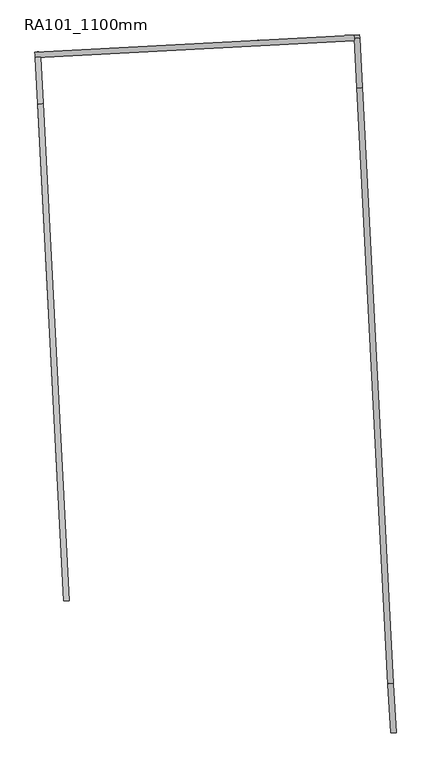
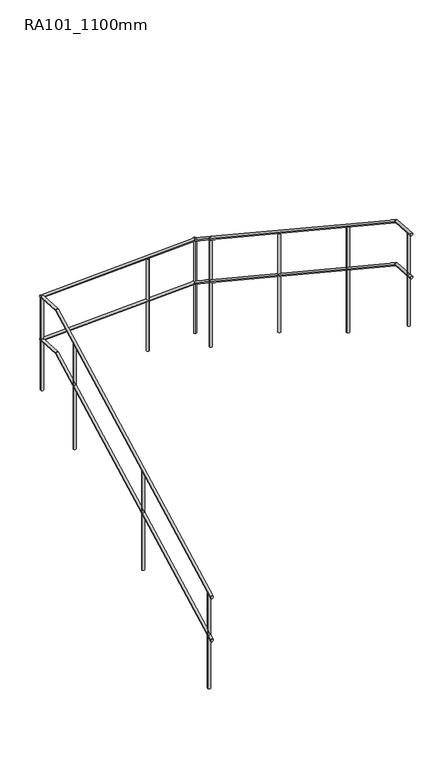
"""IFC4 building model written with IfcOpenShell, lengths in millimetres: railing geometry, RA101_1100mm."""

import ifcopenshell
import ifcopenshell.guid

model = None  # the IFC model being written
_history = None  # IfcOwnerHistory: only IFC2X3 demands one
_inside = {}  # id of a spatial element -> (the spatial element, [elements in it])
_under = {}  # id of a project, library or spatial element -> (it, [spatial elements below it])
_declared = {}  # id of a project -> (the project, [libraries it declares])
_typed = {}  # id of a type object -> (the type object, [elements of that type])
_made_of = {}  # id of a material, layer set ... -> (it, [elements and type objects made of it])


def new_model(schema):
    """Start an empty IFC model of exactly this schema.

    Asked for "IFC4X3", IfcOpenShell would pick the latest addendum, in which some entities
    have other attributes; the version numbers below select the first issue.
    IFC2X3 requires an IfcOwnerHistory on every rooted entity: one is made here for all.
    """
    global model, _history
    if schema == "IFC4X3":
        model = ifcopenshell.file(schema_version=(4, 3, 0, 0))
    else:
        model = ifcopenshell.file(schema=schema)
    _inside.clear()
    _under.clear()
    _declared.clear()
    _typed.clear()
    _made_of.clear()
    _history = None
    if model.schema == "IFC2X3":
        org = make("IfcOrganization", Name="unknown")
        user = make(
            "IfcPersonAndOrganization",
            ThePerson=make("IfcPerson", FamilyName="unknown"),
            TheOrganization=org,
        )
        app = make(
            "IfcApplication",
            ApplicationDeveloper=org,
            Version="unknown",
            ApplicationFullName="unknown",
            ApplicationIdentifier="unknown",
        )
        _history = make(
            "IfcOwnerHistory",
            OwningUser=user,
            OwningApplication=app,
            ChangeAction="ADDED",
            CreationDate=0,
        )
    return model


def make(cls, **values):
    """One entity of the class cls with the attributes given. An attribute that is None is left unset."""
    return model.create_entity(
        cls, **{name: value for name, value in values.items() if value is not None}
    )


def rooted(cls, **values):
    """An entity with a GlobalId (a new one), such as an element, a storey or a relation."""
    return make(cls, GlobalId=ifcopenshell.guid.new(), OwnerHistory=_history, **values)


def si_unit(unit_type, name, prefix=None):
    """IfcSIUnit, for example si_unit("LENGTHUNIT", "METRE", prefix="MILLI")."""
    return make("IfcSIUnit", UnitType=unit_type, Prefix=prefix, Name=name)


def assignment(units):
    """IfcUnitAssignment: the units of a project."""
    return None if units is None else make("IfcUnitAssignment", Units=units)


def point(xyz):
    """IfcCartesianPoint."""
    return None if xyz is None else make("IfcCartesianPoint", Coordinates=xyz)


def direction(xyz):
    """IfcDirection."""
    return None if xyz is None else make("IfcDirection", DirectionRatios=xyz)


def frame(location, z_axis=None, x_axis=None):
    """IfcAxis2Placement3D, a coordinate frame: its origin and axes. An axis left out is left unset."""
    return make(
        "IfcAxis2Placement3D",
        Location=point(location),
        Axis=direction(z_axis),
        RefDirection=direction(x_axis),
    )


def frame_2d(location, x_axis=None):
    """IfcAxis2Placement2D, a coordinate frame in the plane: its origin and x axis."""
    return make(
        "IfcAxis2Placement2D", Location=point(location), RefDirection=direction(x_axis)
    )


def origin():
    """The frame at (0, 0, 0) with its axes left unset."""
    return frame((0.0, 0.0, 0.0))


def place(relative_to, where):
    """IfcLocalPlacement: puts the frame where relative to a parent placement (None: the world)."""
    return make(
        "IfcLocalPlacement", PlacementRelTo=relative_to, RelativePlacement=where
    )


def context(
    kind, dimensions, precision=None, world=None, true_north=None, identifier=None
):
    """IfcGeometricRepresentationContext, for example the 3D "Model" context."""
    return make(
        "IfcGeometricRepresentationContext",
        ContextIdentifier=identifier,
        ContextType=kind,
        CoordinateSpaceDimension=dimensions,
        Precision=precision,
        WorldCoordinateSystem=world,
        TrueNorth=true_north,
    )


def project(units=None, contexts=None):
    """IfcProject with its units and contexts."""
    return rooted(
        "IfcProject",
        Name="project",
        RepresentationContexts=contexts,
        UnitsInContext=assignment(units),
    )


def spatial(cls, under=None, at=None, **own):
    """A site, building, storey or space (cls), placed at a placement, below another one or the project."""
    s = rooted(cls, ObjectPlacement=at, **own)
    if under is not None:
        _under.setdefault(under.id(), (under, []))[1].append(s)
    return s


def circle_curve(where, radius):
    """IfcCircle in the frame where."""
    return make("IfcCircle", Position=where, Radius=radius)


def ellipse_curve(where, semi_axis1, semi_axis2):
    """IfcEllipse in the frame where."""
    return make(
        "IfcEllipse", Position=where, SemiAxis1=semi_axis1, SemiAxis2=semi_axis2
    )


def trimmed(basis, trim1, trim2, sense, master):
    """IfcTrimmedCurve: the piece of a basis curve between two trims."""
    return make(
        "IfcTrimmedCurve",
        BasisCurve=basis,
        Trim1=trim1,
        Trim2=trim2,
        SenseAgreement=sense,
        MasterRepresentation=master,
    )


def segment(curve, same_sense, transition):
    """IfcCompositeCurveSegment."""
    return make(
        "IfcCompositeCurveSegment",
        Transition=transition,
        SameSense=same_sense,
        ParentCurve=curve,
    )


def composite_curve(segments, self_intersect=None):
    """IfcCompositeCurve: segments joined end to end."""
    return make("IfcCompositeCurve", Segments=segments, SelfIntersect=self_intersect)


def outline(outer, holes=None, kind="AREA"):
    """IfcArbitraryClosedProfileDef: a profile drawn as a closed curve; with holes, ...WithVoids."""
    if holes is None:
        return make("IfcArbitraryClosedProfileDef", ProfileType=kind, OuterCurve=outer)
    return make(
        "IfcArbitraryProfileDefWithVoids",
        ProfileType=kind,
        OuterCurve=outer,
        InnerCurves=holes,
    )


def extrude(swept, where, along, depth):
    """IfcExtrudedAreaSolid: the profile swept, set in the frame where, extruded along a direction by depth."""
    return make(
        "IfcExtrudedAreaSolid",
        SweptArea=swept,
        Position=where,
        ExtrudedDirection=direction(along),
        Depth=depth,
    )


def shape(context_of_items, identifier, shape_type, items):
    """IfcShapeRepresentation: the items that make up one representation, for example the "Body"."""
    return make(
        "IfcShapeRepresentation",
        ContextOfItems=context_of_items,
        RepresentationIdentifier=identifier,
        RepresentationType=shape_type,
        Items=items,
    )


def source(mapping_origin, context_of_items, identifier, shape_type, items):
    """IfcRepresentationMap: a shape defined once, which mapped items show again and again."""
    return make(
        "IfcRepresentationMap",
        MappingOrigin=mapping_origin,
        MappedRepresentation=shape(context_of_items, identifier, shape_type, items),
    )


def transform(
    local_origin,
    x_axis=None,
    y_axis=None,
    z_axis=None,
    scale=None,
    scale2=None,
    scale3=None,
    uniform=True,
):
    """IfcCartesianTransformationOperator3D, or its non-uniform kind. x_axis, y_axis, z_axis: its Axis1, 2, 3."""
    if uniform:
        return make(
            "IfcCartesianTransformationOperator3D",
            Axis1=direction(x_axis),
            Axis2=direction(y_axis),
            LocalOrigin=point(local_origin),
            Scale=scale,
            Axis3=direction(z_axis),
        )
    return make(
        "IfcCartesianTransformationOperator3DnonUniform",
        Axis1=direction(x_axis),
        Axis2=direction(y_axis),
        LocalOrigin=point(local_origin),
        Scale=scale,
        Axis3=direction(z_axis),
        Scale2=scale2,
        Scale3=scale3,
    )


def mapped(mapping_source, mapping_target):
    """IfcMappedItem: shows the shape of a source again, moved by a transform."""
    return make(
        "IfcMappedItem", MappingSource=mapping_source, MappingTarget=mapping_target
    )


def made_of(thing, what):
    """Note that an element or type object is made of a material, layer set ...; save() writes the relation."""
    if what is not None:
        _made_of.setdefault(what.id(), (what, []))[1].append(thing)
    return thing


def element(
    cls,
    number,
    at=None,
    inside=None,
    cuts=None,
    type_object=None,
    material=None,
    context=None,
    identifier="Body",
    shape_type=None,
    held_by="IfcProductDefinitionShape",
    body=None,
    shapes=None,
    **own,
):
    """One element of the class cls, such as IfcWall. Its Tag is "e" and its number.

    at: its placement. inside: the storey or other place that contains it. cuts: it is an
    opening in that element (IfcRelVoidsElement). A single representation is given by context,
    identifier, shape_type and body (its items); several are given by shapes. held_by: the class
    of the entity that holds the representations. save() writes the other relations.
    """
    e = rooted(cls, Tag="e%d" % number, ObjectPlacement=at, **own)
    if body is not None:
        shapes = [shape(context, identifier, shape_type, body)]
    if shapes is not None:
        e.Representation = make(held_by, Representations=shapes)
    if inside is not None:
        _inside.setdefault(inside.id(), (inside, []))[1].append(e)
    if cuts is not None:
        rooted(
            "IfcRelVoidsElement", RelatingBuildingElement=cuts, RelatedOpeningElement=e
        )
    if type_object is not None:
        _typed.setdefault(type_object.id(), (type_object, []))[1].append(e)
    return made_of(e, material)


def aggregate(whole, parts):
    """IfcRelAggregates: a whole, such as a stair, and the parts it consists of."""
    return rooted("IfcRelAggregates", RelatingObject=whole, RelatedObjects=parts)


def save(model, path):
    """Write the relations noted so far, then the file.

    IfcRelAggregates (storeys below a building ...), IfcRelContainedInSpatialStructure (elements
    in a storey), IfcRelDefinesByType, IfcRelAssociatesMaterial and IfcRelDeclares: one each for
    every whole, place, type object, material and project.
    """
    for whole, parts in _under.values():
        aggregate(whole, parts)
    for where, things in _inside.values():
        rooted(
            "IfcRelContainedInSpatialStructure",
            RelatedElements=things,
            RelatingStructure=where,
        )
    for kind, things in _typed.values():
        rooted("IfcRelDefinesByType", RelatedObjects=things, RelatingType=kind)
    for what, things in _made_of.values():
        rooted("IfcRelAssociatesMaterial", RelatedObjects=things, RelatingMaterial=what)
    for by, libraries in _declared.values():
        rooted("IfcRelDeclares", RelatingContext=by, RelatedDefinitions=libraries)
    model.write(path)


def plane_surface(at):
    """IfcPlane: the flat surface through the origin of the frame at, square to its z axis."""
    return make("IfcPlane", Position=at)


def cylinder_surface(at, radius):
    """IfcCylindricalSurface: all points at the distance radius from the z axis of the frame at."""
    return make("IfcCylindricalSurface", Position=at, Radius=radius)


def advanced_brep(points, edges, surfaces, faces):
    """IfcAdvancedBrep: a solid bounded by faces that lie on surfaces and meet in shared edges.

    An edge is (start, end): straight between two places in points (the first is 0);
    or (start, end, curve); or (start, end, curve, False) where it runs against its curve.
    A face is (place in surfaces, loops), or (place, loops, False) where it looks against
    its surface's normal. A loop lists edges by number (the first is 1), with a minus sign
    where the edge is run from its end to its start. The first loop is the outer one.
    """
    corners = [point(p) for p in points]
    vertices = [make("IfcVertexPoint", VertexGeometry=c) for c in corners]
    made = []
    for start, end, *more in edges:
        made.append(
            make(
                "IfcEdgeCurve",
                EdgeStart=vertices[start],
                EdgeEnd=vertices[end],
                EdgeGeometry=more[0] if more else make("IfcPolyline", Points=[corners[start], corners[end]]),
                SameSense=more[1] if len(more) > 1 else True,
            )
        )
    hull = []
    for where, loops, *sense in faces:
        bounds = []
        for j, loop in enumerate(loops):
            ring = [make("IfcOrientedEdge", EdgeElement=made[abs(k) - 1], Orientation=k > 0) for k in loop]
            bounds.append(
                make(
                    "IfcFaceOuterBound" if j == 0 else "IfcFaceBound",
                    Bound=make("IfcEdgeLoop", EdgeList=ring),
                    Orientation=True,
                )
            )
        hull.append(make("IfcAdvancedFace", Bounds=bounds, FaceSurface=surfaces[where], SameSense=sense[0] if sense else True))
    return make("IfcAdvancedBrep", Outer=make("IfcClosedShell", CfsFaces=hull))


def ra101_1100mm_54c19647(model_context):
    return source(origin(), model_context, "Body", "SolidModel", [
        advanced_brep(
        [(22896.1789103, 12534.7141331, 457.1248327), (22926.1377964, 12536.2842117, 457.1248327), (22754.6396676, 15235.4437699, 2210.0), (22784.5985536, 15237.0138486, 2210.0), (22741.5052252, 15486.0638601, 2210.0), (22771.4641113, 15487.6339388, 2210.0)],
        [
            (0, 1, ellipse_curve(frame((22911.1583533, 12535.4991724, 457.1248327), z_axis=(0.05233595624294174, -0.998629534754574, 0.0), x_axis=(0.0, 0.0, -0.9999999999999999)), 17.8751673, 15.0)),
            (1, 0, ellipse_curve(frame((22911.1583533, 12535.4991724, 457.1248327), z_axis=(0.05233595624294174, -0.998629534754574, 0.0), x_axis=(0.0, 0.0, -0.9999999999999999)), 17.8751673, 15.0)),
            (0, 2),
            (2, 3, ellipse_curve(frame((22769.6191106, 15236.2288092, 2210.0), z_axis=(0.05018733030882238, -0.9576313096148807, -0.28359038545367066), x_axis=(-0.014841974004015643, 0.28320173468646914, -0.9589455111101144)), 15.6421818, 15.0)),
            (3, 1),
            (3, 2, ellipse_curve(frame((22769.6191106, 15236.2288092, 2210.0), z_axis=(0.05018733030882238, -0.9576313096148807, -0.28359038545367066), x_axis=(-0.014841974004015643, 0.28320173468646914, -0.9589455111101144)), 15.6421818, 15.0)),
            (4, 5, circle_curve(frame((22756.4846683, 15486.8488994, 2210.0), z_axis=(-0.05233595624293797, 0.9986295347545743, 0.0), x_axis=(0.9986295347545743, 0.05233595624293797, 0.0)), 15.0)),
            (5, 4, circle_curve(frame((22756.4846683, 15486.8488994, 2210.0), z_axis=(-0.05233595624293797, 0.9986295347545743, 0.0), x_axis=(0.9986295347545743, 0.05233595624293797, 0.0)), 15.0)),
            (2, 4),
            (5, 3),
        ],
        [
            plane_surface(frame((22911.1583533, 12535.4991724, 475.0), z_axis=(0.05233595624294174, -0.998629534754574, 0.0), x_axis=(0.998629534754574, 0.05233595624294174, 0.0))),
            cylinder_surface(frame((22910.731374, 12543.6464234, 462.4127052), z_axis=(0.04391787398555367, -0.8380029565528062, -0.5438954542495689), x_axis=(0.998629534754574, 0.052335956242941746, 0.0)), 15.0),
            plane_surface(frame((22756.4846683, 15486.8488994, 2225.0), z_axis=(-0.05233595624294184, 0.998629534754574, 0.0), x_axis=(0.998629534754574, 0.05233595624294184, 0.0))),
            cylinder_surface(frame((22769.8512715, 15231.7989162, 2210.0), z_axis=(0.05233595624293797, -0.9986295347545743, 0.0), x_axis=(0.9986295347545743, 0.05233595624293797, 0.0)), 15.0),
        ],
        [
            (0, [[1, 2]]),
            (1, [[-1, 3, 4, 5]]),
            (1, [[-2, -5, 6, -3]]),
            (2, [[7, 8]]),
            (3, [[-4, 9, -8, 10]]),
            (3, [[-6, -10, -7, -9]]),
        ],
    ),
        advanced_brep(
        [(22739.9351465, 15516.0227461, 2210.0), (22741.5052252, 15486.0638601, 2210.0), (24475.8528668, 15606.9983388, 2210.0), (24477.4229455, 15577.0394528, 2210.0)],
        [
            (0, 1, circle_curve(frame((22740.7201859, 15501.0433031, 2210.0), z_axis=(-0.998629534754574, -0.05233595624294185, 0.0), x_axis=(0.05233595624294185, -0.998629534754574, 0.0)), 15.0)),
            (1, 0, circle_curve(frame((22740.7201859, 15501.0433031, 2210.0), z_axis=(-0.998629534754574, -0.05233595624294185, 0.0), x_axis=(0.05233595624294185, -0.998629534754574, 0.0)), 15.0)),
            (2, 3, circle_curve(frame((24476.6379061, 15592.0188958, 2210.0), z_axis=(0.998629534754574, 0.05233595624294185, 0.0), x_axis=(0.05233595624294185, -0.998629534754574, 0.0)), 15.0)),
            (3, 2, circle_curve(frame((24476.6379061, 15592.0188958, 2210.0), z_axis=(0.998629534754574, 0.05233595624294185, 0.0), x_axis=(0.05233595624294185, -0.998629534754574, 0.0)), 15.0)),
            (0, 2),
            (3, 1),
        ],
        [
            plane_surface(frame((22740.7201859, 15501.0433031, 2225.0), z_axis=(-0.9986295347545743, -0.052335956242937944, 0.0), x_axis=(0.052335956242937944, -0.9986295347545743, 0.0))),
            plane_surface(frame((24476.6379061, 15592.0188958, 2225.0), z_axis=(0.9986295347545743, 0.052335956242937104, 0.0), x_axis=(0.052335956242937104, -0.9986295347545743, 0.0))),
            cylinder_surface(frame((22740.7201859, 15501.0433031, 2210.0), z_axis=(-0.998629534754574, -0.05233595624294185, 0.0), x_axis=(0.05233595624294185, -0.998629534754574, 0.0)), 15.0),
        ],
        [
            (0, [[1, 2]]),
            (1, [[3, 4]]),
            (2, [[-1, 5, -4, 6]]),
            (2, [[-2, -6, -3, -5]]),
        ],
    ),
        advanced_brep(
        [(24505.8117528, 15608.5684175, 2210.0), (24475.8528668, 15606.9983388, 2210.0), (24506.8498874, 15588.7596297, 2210.0), (24476.8910014, 15587.189551, 2210.0), (24520.7484348, 15323.5595483, 2382.1248327), (24490.7895487, 15321.9894696, 2382.1248327)],
        [
            (0, 1, circle_curve(frame((24490.8323098, 15607.7833782, 2210.0), z_axis=(-0.052335956242937104, 0.9986295347545743, 0.0), x_axis=(-0.9986295347545743, -0.052335956242937104, 0.0)), 15.0)),
            (1, 0, circle_curve(frame((24490.8323098, 15607.7833782, 2210.0), z_axis=(-0.052335956242937104, 0.9986295347545743, 0.0), x_axis=(-0.9986295347545743, -0.052335956242937104, 0.0)), 15.0)),
            (0, 2),
            (2, 3, ellipse_curve(frame((24491.8704444, 15587.9745903, 2210.0), z_axis=(-0.050187330308819895, 0.9576313096148807, -0.28359038545367116), x_axis=(-0.014841974004020982, 0.2832017346864703, 0.9589455111101142)), 15.6421818, 15.0)),
            (3, 1),
            (3, 2, ellipse_curve(frame((24491.8704444, 15587.9745903, 2210.0), z_axis=(-0.050187330308819895, 0.9576313096148807, -0.28359038545367116), x_axis=(-0.014841974004020982, 0.2832017346864703, 0.9589455111101142)), 15.6421818, 15.0)),
            (4, 5, ellipse_curve(frame((24505.7689917, 15322.774509, 2382.1248327), z_axis=(0.052335956242937104, -0.9986295347545743, 0.0), x_axis=(0.0, 0.0, -1.0)), 17.8751673, 15.0)),
            (5, 4, ellipse_curve(frame((24505.7689917, 15322.774509, 2382.1248327), z_axis=(0.052335956242937104, -0.9986295347545743, 0.0), x_axis=(0.0, 0.0, -1.0)), 17.8751673, 15.0)),
            (2, 4),
            (5, 3),
        ],
        [
            plane_surface(frame((24490.8323098, 15607.7833782, 2225.0), z_axis=(-0.05233595624294184, 0.998629534754574, 0.0), x_axis=(0.998629534754574, 0.05233595624294184, 0.0))),
            cylinder_surface(frame((24490.8323098, 15607.7833782, 2210.0), z_axis=(-0.052335956242937104, 0.9986295347545743, 0.0), x_axis=(-0.9986295347545743, -0.052335956242937104, 0.0)), 15.0),
            plane_surface(frame((24505.7689917, 15322.774509, 2400.0), z_axis=(0.052335956242937104, -0.9986295347545743, 0.0), x_axis=(0.9986295347545743, 0.052335956242937104, 0.0))),
            cylinder_surface(frame((24492.0652629, 15584.2572324, 2212.4127052), z_axis=(-0.04391787398554974, 0.8380029565528057, -0.5438954542495701), x_axis=(-0.9986295347545743, -0.0523359562429371, 0.0)), 15.0),
        ],
        [
            (0, [[1, 2]]),
            (1, [[-1, 3, 4, 5]]),
            (1, [[-2, -5, 6, -3]]),
            (2, [[7, 8]]),
            (3, [[-4, 9, -8, 10]]),
            (3, [[-6, -10, -7, -9]]),
        ],
    ),
        advanced_brep(
        [(24520.7484348, 15323.5595483, 2382.1248327), (24490.7895487, 15321.9894696, 2382.1248327), (24690.5490938, 12083.5699627, 4485.0), (24660.5902078, 12081.999884, 4485.0), (24704.4476412, 11818.3698813, 4485.0), (24674.4887551, 11816.7998026, 4485.0)],
        [
            (0, 1, ellipse_curve(frame((24505.7689917, 15322.774509, 2382.1248327), z_axis=(-0.05233595624294191, 0.998629534754574, 0.0), x_axis=(0.0, 0.0, -1.0)), 17.8751673, 15.0)),
            (1, 0, ellipse_curve(frame((24505.7689917, 15322.774509, 2382.1248327), z_axis=(-0.05233595624294191, 0.998629534754574, 0.0), x_axis=(0.0, 0.0, -1.0)), 17.8751673, 15.0)),
            (0, 2),
            (2, 3, ellipse_curve(frame((24675.5696508, 12082.7849234, 4485.0), z_axis=(-0.05018733030882025, 0.9576313096148807, -0.28359038545367127), x_axis=(0.014841974004007963, -0.28320173468647103, -0.9589455111101143)), 15.6421818, 15.0)),
            (3, 1),
            (3, 2, ellipse_curve(frame((24675.5696508, 12082.7849234, 4485.0), z_axis=(-0.05018733030882025, 0.9576313096148807, -0.28359038545367127), x_axis=(0.014841974004007963, -0.28320173468647103, -0.9589455111101143)), 15.6421818, 15.0)),
            (4, 5, circle_curve(frame((24689.4681982, 11817.584842, 4485.0), z_axis=(0.05233595624293375, -0.9986295347545745, 0.0), x_axis=(-0.9986295347545745, -0.05233595624293375, 0.0)), 15.0)),
            (5, 4, circle_curve(frame((24689.4681982, 11817.584842, 4485.0), z_axis=(0.05233595624293375, -0.9986295347545745, 0.0), x_axis=(-0.9986295347545745, -0.05233595624293375, 0.0)), 15.0)),
            (2, 4),
            (5, 3),
        ],
        [
            plane_surface(frame((24505.7689917, 15322.774509, 2400.0), z_axis=(-0.05233595624294191, 0.998629534754574, 0.0), x_axis=(0.998629534754574, 0.05233595624294191, 0.0))),
            cylinder_surface(frame((24506.1959711, 15314.627258, 2387.4127052), z_axis=(-0.04391787398555378, 0.8380029565528053, -0.5438954542495702), x_axis=(-0.998629534754574, -0.052335956242941926, 0.0)), 15.0),
            plane_surface(frame((24689.4681982, 11817.584842, 4500.0), z_axis=(0.05233595624293375, -0.9986295347545745, 0.0), x_axis=(0.9986295347545745, 0.05233595624293375, 0.0))),
            cylinder_surface(frame((24675.33749, 12087.2148164, 4485.0), z_axis=(-0.05233595624293375, 0.9986295347545745, 0.0), x_axis=(-0.9986295347545745, -0.05233595624293375, 0.0)), 15.0),
        ],
        [
            (0, [[1, 2]]),
            (1, [[-1, 3, 4, 5]]),
            (1, [[-2, -5, 6, -3]]),
            (2, [[7, 8]]),
            (3, [[-4, 9, -8, 10]]),
            (3, [[-6, -10, -7, -9]]),
        ],
    ),
        advanced_brep(
        [(22896.1789103, 12534.7141331, 957.1248327), (22926.1377964, 12536.2842117, 957.1248327), (22754.6396676, 15235.4437699, 2710.0), (22784.5985536, 15237.0138486, 2710.0), (22741.5052252, 15486.0638601, 2710.0), (22771.4641113, 15487.6339388, 2710.0)],
        [
            (0, 1, ellipse_curve(frame((22911.1583533, 12535.4991724, 957.1248327), z_axis=(0.05233595624294174, -0.998629534754574, 0.0), x_axis=(0.0, 0.0, -0.9999999999999999)), 17.8751673, 15.0)),
            (1, 0, ellipse_curve(frame((22911.1583533, 12535.4991724, 957.1248327), z_axis=(0.05233595624294174, -0.998629534754574, 0.0), x_axis=(0.0, 0.0, -0.9999999999999999)), 17.8751673, 15.0)),
            (0, 2),
            (2, 3, ellipse_curve(frame((22769.6191106, 15236.2288092, 2710.0), z_axis=(0.05018733030882238, -0.9576313096148807, -0.28359038545367066), x_axis=(-0.014841974004015643, 0.28320173468646914, -0.9589455111101144)), 15.6421818, 15.0)),
            (3, 1),
            (3, 2, ellipse_curve(frame((22769.6191106, 15236.2288092, 2710.0), z_axis=(0.05018733030882238, -0.9576313096148807, -0.28359038545367066), x_axis=(-0.014841974004015643, 0.28320173468646914, -0.9589455111101144)), 15.6421818, 15.0)),
            (4, 5, circle_curve(frame((22756.4846683, 15486.8488994, 2710.0), z_axis=(-0.05233595624293797, 0.9986295347545743, 0.0), x_axis=(0.9986295347545743, 0.05233595624293797, 0.0)), 15.0)),
            (5, 4, circle_curve(frame((22756.4846683, 15486.8488994, 2710.0), z_axis=(-0.05233595624293797, 0.9986295347545743, 0.0), x_axis=(0.9986295347545743, 0.05233595624293797, 0.0)), 15.0)),
            (2, 4),
            (5, 3),
        ],
        [
            plane_surface(frame((22911.1583533, 12535.4991724, 975.0), z_axis=(0.05233595624294174, -0.998629534754574, 0.0), x_axis=(0.998629534754574, 0.05233595624294174, 0.0))),
            cylinder_surface(frame((22910.731374, 12543.6464234, 962.4127052), z_axis=(0.04391787398555367, -0.8380029565528062, -0.5438954542495689), x_axis=(0.998629534754574, 0.052335956242941746, 0.0)), 15.0),
            plane_surface(frame((22756.4846683, 15486.8488994, 2725.0), z_axis=(-0.05233595624294184, 0.998629534754574, 0.0), x_axis=(0.998629534754574, 0.05233595624294184, 0.0))),
            cylinder_surface(frame((22769.8512715, 15231.7989162, 2710.0), z_axis=(0.05233595624293797, -0.9986295347545743, 0.0), x_axis=(0.9986295347545743, 0.05233595624293797, 0.0)), 15.0),
        ],
        [
            (0, [[1, 2]]),
            (1, [[-1, 3, 4, 5]]),
            (1, [[-2, -5, 6, -3]]),
            (2, [[7, 8]]),
            (3, [[-4, 9, -8, 10]]),
            (3, [[-6, -10, -7, -9]]),
        ],
    ),
        advanced_brep(
        [(22739.9351465, 15516.0227461, 2710.0), (22741.5052252, 15486.0638601, 2710.0), (24475.8528668, 15606.9983388, 2710.0), (24477.4229455, 15577.0394528, 2710.0)],
        [
            (0, 1, circle_curve(frame((22740.7201859, 15501.0433031, 2710.0), z_axis=(-0.998629534754574, -0.05233595624294185, 0.0), x_axis=(0.05233595624294185, -0.998629534754574, 0.0)), 15.0)),
            (1, 0, circle_curve(frame((22740.7201859, 15501.0433031, 2710.0), z_axis=(-0.998629534754574, -0.05233595624294185, 0.0), x_axis=(0.05233595624294185, -0.998629534754574, 0.0)), 15.0)),
            (2, 3, circle_curve(frame((24476.6379061, 15592.0188958, 2710.0), z_axis=(0.998629534754574, 0.05233595624294185, 0.0), x_axis=(0.05233595624294185, -0.998629534754574, 0.0)), 15.0)),
            (3, 2, circle_curve(frame((24476.6379061, 15592.0188958, 2710.0), z_axis=(0.998629534754574, 0.05233595624294185, 0.0), x_axis=(0.05233595624294185, -0.998629534754574, 0.0)), 15.0)),
            (0, 2),
            (3, 1),
        ],
        [
            plane_surface(frame((22740.7201859, 15501.0433031, 2725.0), z_axis=(-0.9986295347545743, -0.052335956242937944, 0.0), x_axis=(0.052335956242937944, -0.9986295347545743, 0.0))),
            plane_surface(frame((24476.6379061, 15592.0188958, 2725.0), z_axis=(0.9986295347545743, 0.052335956242937104, 0.0), x_axis=(0.052335956242937104, -0.9986295347545743, 0.0))),
            cylinder_surface(frame((22740.7201859, 15501.0433031, 2710.0), z_axis=(-0.998629534754574, -0.05233595624294185, 0.0), x_axis=(0.05233595624294185, -0.998629534754574, 0.0)), 15.0),
        ],
        [
            (0, [[1, 2]]),
            (1, [[3, 4]]),
            (2, [[-1, 5, -4, 6]]),
            (2, [[-2, -6, -3, -5]]),
        ],
    ),
        advanced_brep(
        [(24505.8117528, 15608.5684175, 2710.0), (24475.8528668, 15606.9983388, 2710.0), (24506.8498874, 15588.7596297, 2710.0), (24476.8910014, 15587.189551, 2710.0), (24520.7484348, 15323.5595483, 2882.1248327), (24490.7895487, 15321.9894696, 2882.1248327)],
        [
            (0, 1, circle_curve(frame((24490.8323098, 15607.7833782, 2710.0), z_axis=(-0.052335956242937104, 0.9986295347545743, 0.0), x_axis=(-0.9986295347545743, -0.052335956242937104, 0.0)), 15.0)),
            (1, 0, circle_curve(frame((24490.8323098, 15607.7833782, 2710.0), z_axis=(-0.052335956242937104, 0.9986295347545743, 0.0), x_axis=(-0.9986295347545743, -0.052335956242937104, 0.0)), 15.0)),
            (0, 2),
            (2, 3, ellipse_curve(frame((24491.8704444, 15587.9745903, 2710.0), z_axis=(-0.050187330308819895, 0.9576313096148807, -0.28359038545367116), x_axis=(-0.014841974004020982, 0.2832017346864703, 0.9589455111101142)), 15.6421818, 15.0)),
            (3, 1),
            (3, 2, ellipse_curve(frame((24491.8704444, 15587.9745903, 2710.0), z_axis=(-0.050187330308819895, 0.9576313096148807, -0.28359038545367116), x_axis=(-0.014841974004020982, 0.2832017346864703, 0.9589455111101142)), 15.6421818, 15.0)),
            (4, 5, ellipse_curve(frame((24505.7689917, 15322.774509, 2882.1248327), z_axis=(0.052335956242937104, -0.9986295347545743, 0.0), x_axis=(0.0, 0.0, -1.0)), 17.8751673, 15.0)),
            (5, 4, ellipse_curve(frame((24505.7689917, 15322.774509, 2882.1248327), z_axis=(0.052335956242937104, -0.9986295347545743, 0.0), x_axis=(0.0, 0.0, -1.0)), 17.8751673, 15.0)),
            (2, 4),
            (5, 3),
        ],
        [
            plane_surface(frame((24490.8323098, 15607.7833782, 2725.0), z_axis=(-0.05233595624294184, 0.998629534754574, 0.0), x_axis=(0.998629534754574, 0.05233595624294184, 0.0))),
            cylinder_surface(frame((24490.8323098, 15607.7833782, 2710.0), z_axis=(-0.052335956242937104, 0.9986295347545743, 0.0), x_axis=(-0.9986295347545743, -0.052335956242937104, 0.0)), 15.0),
            plane_surface(frame((24505.7689917, 15322.774509, 2900.0), z_axis=(0.052335956242937104, -0.9986295347545743, 0.0), x_axis=(0.9986295347545743, 0.052335956242937104, 0.0))),
            cylinder_surface(frame((24492.0652629, 15584.2572324, 2712.4127052), z_axis=(-0.04391787398554974, 0.8380029565528057, -0.5438954542495701), x_axis=(-0.9986295347545743, -0.0523359562429371, 0.0)), 15.0),
        ],
        [
            (0, [[1, 2]]),
            (1, [[-1, 3, 4, 5]]),
            (1, [[-2, -5, 6, -3]]),
            (2, [[7, 8]]),
            (3, [[-4, 9, -8, 10]]),
            (3, [[-6, -10, -7, -9]]),
        ],
    ),
        advanced_brep(
        [(24520.7484348, 15323.5595483, 2882.1248327), (24490.7895487, 15321.9894696, 2882.1248327), (24690.5490938, 12083.5699627, 4985.0), (24660.5902078, 12081.999884, 4985.0), (24704.4476412, 11818.3698813, 4985.0), (24674.4887551, 11816.7998026, 4985.0)],
        [
            (0, 1, ellipse_curve(frame((24505.7689917, 15322.774509, 2882.1248327), z_axis=(-0.05233595624294191, 0.998629534754574, 0.0), x_axis=(0.0, 0.0, -1.0)), 17.8751673, 15.0)),
            (1, 0, ellipse_curve(frame((24505.7689917, 15322.774509, 2882.1248327), z_axis=(-0.05233595624294191, 0.998629534754574, 0.0), x_axis=(0.0, 0.0, -1.0)), 17.8751673, 15.0)),
            (0, 2),
            (2, 3, ellipse_curve(frame((24675.5696508, 12082.7849234, 4985.0), z_axis=(-0.05018733030882025, 0.9576313096148807, -0.28359038545367127), x_axis=(0.014841974004007963, -0.28320173468647103, -0.9589455111101143)), 15.6421818, 15.0)),
            (3, 1),
            (3, 2, ellipse_curve(frame((24675.5696508, 12082.7849234, 4985.0), z_axis=(-0.05018733030882025, 0.9576313096148807, -0.28359038545367127), x_axis=(0.014841974004007963, -0.28320173468647103, -0.9589455111101143)), 15.6421818, 15.0)),
            (4, 5, circle_curve(frame((24689.4681982, 11817.584842, 4985.0), z_axis=(0.05233595624293375, -0.9986295347545745, 0.0), x_axis=(-0.9986295347545745, -0.05233595624293375, 0.0)), 15.0)),
            (5, 4, circle_curve(frame((24689.4681982, 11817.584842, 4985.0), z_axis=(0.05233595624293375, -0.9986295347545745, 0.0), x_axis=(-0.9986295347545745, -0.05233595624293375, 0.0)), 15.0)),
            (2, 4),
            (5, 3),
        ],
        [
            plane_surface(frame((24505.7689917, 15322.774509, 2900.0), z_axis=(-0.05233595624294191, 0.998629534754574, 0.0), x_axis=(0.998629534754574, 0.05233595624294191, 0.0))),
            cylinder_surface(frame((24506.1959711, 15314.627258, 2887.4127052), z_axis=(-0.04391787398555378, 0.8380029565528053, -0.5438954542495702), x_axis=(-0.998629534754574, -0.052335956242941926, 0.0)), 15.0),
            plane_surface(frame((24689.4681982, 11817.584842, 5000.0), z_axis=(0.05233595624293375, -0.9986295347545745, 0.0), x_axis=(0.9986295347545745, 0.05233595624293375, 0.0))),
            cylinder_surface(frame((24675.33749, 12087.2148164, 4985.0), z_axis=(-0.05233595624293375, 0.9986295347545745, 0.0), x_axis=(-0.9986295347545745, -0.05233595624293375, 0.0)), 15.0),
        ],
        [
            (0, [[1, 2]]),
            (1, [[-1, 3, 4, 5]]),
            (1, [[-2, -5, 6, -3]]),
            (2, [[7, 8]]),
            (3, [[-4, 9, -8, 10]]),
            (3, [[-6, -10, -7, -9]]),
        ],
    ),
        extrude(outline(composite_curve([segment(trimmed(circle_curve(frame_2d((24631.3752867, 12926.0636256)), 15.0), [point((24616.3958437, 12925.2785862))], [point((24646.3547297, 12926.8486649))], False, "CARTESIAN"), True, "CONTINUOUS"), segment(trimmed(circle_curve(frame_2d((24631.3752867, 12926.0636256)), 15.0), [point((24646.3547297, 12926.8486649))], [point((24616.3958437, 12925.2785862))], False, "CARTESIAN"), True, "CONTINUOUS")], self_intersect=False)), frame((0.0, 0.0, 3200.0), z_axis=(0.0, 0.0, 1.0), x_axis=(1.0, 0.0, 0.0)), (0.0, 0.0, 1.0), 1225.5555556),
        extrude(outline(composite_curve([segment(trimmed(circle_curve(frame_2d((24568.5721392, 14124.4190673)), 15.0), [point((24553.5926962, 14123.6340279))], [point((24583.5515823, 14125.2041066))], False, "CARTESIAN"), True, "CONTINUOUS"), segment(trimmed(circle_curve(frame_2d((24568.5721392, 14124.4190673)), 15.0), [point((24583.5515823, 14125.2041066))], [point((24553.5926962, 14123.6340279))], False, "CARTESIAN"), True, "CONTINUOUS")], self_intersect=False)), frame((0.0, 0.0, 2500.0), z_axis=(0.0, 0.0, 1.0), x_axis=(1.0, 0.0, 0.0)), (0.0, 0.0, 1.0), 1147.7777778),
        extrude(outline(composite_curve([segment(trimmed(circle_curve(frame_2d((23954.0550706, 15564.6314899)), 15.0), [point((23954.84011, 15549.6520469))], [point((23953.2700313, 15579.6109329))], False, "CARTESIAN"), True, "CONTINUOUS"), segment(trimmed(circle_curve(frame_2d((23954.0550706, 15564.6314899)), 15.0), [point((23953.2700313, 15579.6109329))], [point((23954.84011, 15549.6520469))], False, "CARTESIAN"), True, "CONTINUOUS")], self_intersect=False)), frame((0.0, 0.0, 1625.0), z_axis=(0.0, 0.0, 1.0), x_axis=(1.0, 0.0, 0.0)), (0.0, 0.0, 1.0), 1070.0),
        extrude(outline(composite_curve([segment(trimmed(circle_curve(frame_2d((22785.5520583, 14932.2100558)), 15.0), [point((22800.5315014, 14932.9950952))], [point((22770.5726153, 14931.4250165))], False, "CARTESIAN"), True, "CONTINUOUS"), segment(trimmed(circle_curve(frame_2d((22785.5520583, 14932.2100558)), 15.0), [point((22770.5726153, 14931.4250165))], [point((22800.5315014, 14932.9950952))], False, "CARTESIAN"), True, "CONTINUOUS")], self_intersect=False)), frame((0.0, 0.0, 1275.0), z_axis=(0.0, 0.0, 1.0), x_axis=(1.0, 0.0, 0.0)), (0.0, 0.0, 1.0), 1225.5555556),
        extrude(outline(composite_curve([segment(trimmed(circle_curve(frame_2d((22848.3552058, 13733.8546141)), 15.0), [point((22863.3346489, 13734.6396534))], [point((22833.3757628, 13733.0695748))], False, "CARTESIAN"), True, "CONTINUOUS"), segment(trimmed(circle_curve(frame_2d((22848.3552058, 13733.8546141)), 15.0), [point((22833.3757628, 13733.0695748))], [point((22863.3346489, 13734.6396534))], False, "CARTESIAN"), True, "CONTINUOUS")], self_intersect=False)), frame((0.0, 0.0, 575.0), z_axis=(0.0, 0.0, 1.0), x_axis=(1.0, 0.0, 0.0)), (0.0, 0.0, 1.0), 1147.7777778),
        extrude(outline(composite_curve([segment(trimmed(circle_curve(frame_2d((24505.7689917, 15322.774509)), 15.0), [point((24490.7895487, 15321.9894696))], [point((24520.7484348, 15323.5595483))], False, "CARTESIAN"), True, "CONTINUOUS"), segment(trimmed(circle_curve(frame_2d((24505.7689917, 15322.774509)), 15.0), [point((24520.7484348, 15323.5595483))], [point((24490.7895487, 15321.9894696))], False, "CARTESIAN"), True, "CONTINUOUS")], self_intersect=False)), frame((0.0, 0.0, 1625.0), z_axis=(0.0, 0.0, 1.0), x_axis=(1.0, 0.0, 0.0)), (0.0, 0.0, 1.0), 1245.0),
        extrude(outline(composite_curve([segment(trimmed(circle_curve(frame_2d((24491.6173492, 15592.8039352)), 15.0), [point((24492.4023885, 15577.8244921))], [point((24490.8323098, 15607.7833782))], False, "CARTESIAN"), True, "CONTINUOUS"), segment(trimmed(circle_curve(frame_2d((24491.6173492, 15592.8039352)), 15.0), [point((24490.8323098, 15607.7833782))], [point((24492.4023885, 15577.8244921))], False, "CARTESIAN"), True, "CONTINUOUS")], self_intersect=False)), frame((0.0, 0.0, 1625.0), z_axis=(0.0, 0.0, 1.0), x_axis=(1.0, 0.0, 0.0)), (0.0, 0.0, 1.0), 1070.0),
        extrude(outline(composite_curve([segment(trimmed(circle_curve(frame_2d((22755.6996289, 15501.8283424)), 15.0), [point((22770.6790719, 15502.6133818))], [point((22740.7201859, 15501.0433031))], False, "CARTESIAN"), True, "CONTINUOUS"), segment(trimmed(circle_curve(frame_2d((22755.6996289, 15501.8283424)), 15.0), [point((22740.7201859, 15501.0433031))], [point((22770.6790719, 15502.6133818))], False, "CARTESIAN"), True, "CONTINUOUS")], self_intersect=False)), frame((0.0, 0.0, 1625.0), z_axis=(0.0, 0.0, 1.0), x_axis=(1.0, 0.0, 0.0)), (0.0, 0.0, 1.0), 1070.0),
        extrude(outline(composite_curve([segment(trimmed(circle_curve(frame_2d((24686.8514003, 11867.5163187)), 15.0), [point((24671.8719573, 11866.7312794))], [point((24701.8308434, 11868.3013581))], False, "CARTESIAN"), True, "CONTINUOUS"), segment(trimmed(circle_curve(frame_2d((24686.8514003, 11867.5163187)), 15.0), [point((24701.8308434, 11868.3013581))], [point((24671.8719573, 11866.7312794))], False, "CARTESIAN"), True, "CONTINUOUS")], self_intersect=False)), frame((0.0, 0.0, 3900.0), z_axis=(0.0, 0.0, 1.0), x_axis=(1.0, 0.0, 0.0)), (0.0, 0.0, 1.0), 1070.0),
        extrude(outline(composite_curve([segment(trimmed(circle_curve(frame_2d((22908.5415555, 12585.4306491)), 15.0), [point((22923.5209985, 12586.2156885))], [point((22893.5621125, 12584.6456098))], False, "CARTESIAN"), True, "CONTINUOUS"), segment(trimmed(circle_curve(frame_2d((22908.5415555, 12585.4306491)), 15.0), [point((22893.5621125, 12584.6456098))], [point((22923.5209985, 12586.2156885))], False, "CARTESIAN"), True, "CONTINUOUS")], self_intersect=False)), frame((0.0, 0.0, -125.0), z_axis=(0.0, 0.0, 1.0), x_axis=(1.0, 0.0, 0.0)), (0.0, 0.0, 1.0), 1102.4074074),
    ])


if __name__ == "__main__":
    model = new_model("IFC4")
    model_context = context("Model", 3, world=origin())
    ifc_project = project(units=[si_unit("LENGTHUNIT", "METRE", prefix="MILLI")], contexts=[model_context])
    site = spatial("IfcSite", under=ifc_project)
    building = spatial("IfcBuilding", under=site)
    placement = place(None, origin())
    ra101_1100mm_shape = ra101_1100mm_54c19647(model_context)
    element("IfcRailing", 1, ObjectType="RA101_1100mm", at=placement, inside=building, context=model_context, shape_type="MappedRepresentation", body=[
        mapped(ra101_1100mm_shape, transform((0.0, 0.0, 0.0), x_axis=(1.0, 0.0, 0.0), y_axis=(0.0, 1.0, 0.0), z_axis=(0.0, 0.0, 1.0))),
    ])
    save(model, "model.ifc")

# Revit data of these elements
# Project information
#   Building Name = "MAIN GATE SECURITY BUILDING"
#   Project Status = "Project Status"
#   Client Name = "현대엔지니어링"
#   Project Address = "서울시 종로구 율곡로 75(계동)"
#   Project Name = "Therma Visayas Energy Project"
#   Project Number = "-"
